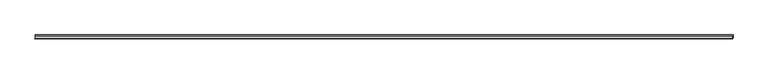
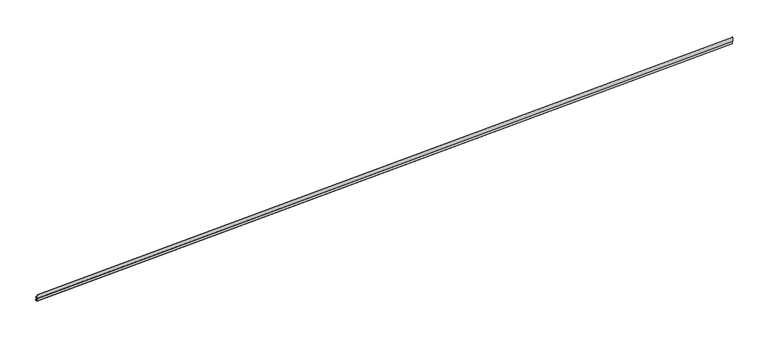
"""IFC4 building model written with IfcOpenShell, lengths in millimetres: proxy geometry, Generic Models 2:Generic Models 2:310765:Generic Models 2:310765 : Generic Models 2:Generic Models 2:310765:197 : Generic Models 2:Generic Models 2:310765:Generic Models 2:310765 : Generic Models 2:Generic Models 2:310765:300385."""

from ifc_helpers import new_model, si_unit, frame, origin, place, context, project, spatial, polyline, outline, extrude, source, transform, mapped, element, save


def generic_models_54930a4b(model_context):
    return source(origin(), model_context, "Body", "SweptSolid", [
        extrude(outline(polyline([(-6.35, 0.0), (-6.35, -90.4875), (-7.9375, -90.4875), (-7.9375, -1.5874999), (-72.095064, -1.5874999), (-72.095064, 11.1125), (-53.045064, 11.1125), (-53.045064, 9.525), (-70.507564, 9.525), (-70.507564, 0.0), (-6.35, 0.0)])), frame((563227.6289933, -578787.9663841, 4134.5272352), z_axis=(0.9991330730923568, 0.0, 0.04163054471206784), x_axis=(0.0, -1.0, 0.0)), (0.0, 0.0, 1.0), 15852.9020761),
        extrude(outline(polyline([(-48.7009311, 5.5562501), (-48.7009311, 56.35625), (-47.1134311, 56.35625), (-47.1134311, 3.96875), (-67.5700628, 3.96875), (-67.5700628, 5.5562501), (-48.7009311, 5.5562501)])), frame((563227.6289933, -578787.9663841, 4134.5272352), z_axis=(0.9991330730923568, 0.0, 0.04163054471206784), x_axis=(0.0, -1.0, 0.0)), (0.0, 0.0, 1.0), 15852.9020761),
        extrude(outline(polyline([(-36.5125, 89.69375), (-36.5125, 26.1937501), (-38.1, 26.1937501), (-38.1, 88.10625), (-97.7325628, 88.10625), (-97.7325628, 89.69375), (-36.5125, 89.69375)])), frame((563227.6289933, -578787.9663841, 4134.5272352), z_axis=(0.9991330730923568, 0.0, 0.04163054471206784), x_axis=(0.0, -1.0, 0.0)), (0.0, 0.0, 1.0), 15852.9020761),
    ])


if __name__ == "__main__":
    model = new_model("IFC4")
    model_context = context("Model", 3, world=origin())
    ifc_project = project(units=[si_unit("LENGTHUNIT", "METRE", prefix="MILLI")], contexts=[model_context])
    site = spatial("IfcSite", under=ifc_project)
    building = spatial("IfcBuilding", under=site)
    placement = place(None, origin())
    generic_models_shape = generic_models_54930a4b(model_context)
    element("IfcBuildingElementProxy", 1, Name="Generic Models 2:Generic Models 2:310765:Generic Models 2:310765 : Generic Models 2:Generic Models 2:310765:197 : Generic Models 2:Generic Models 2:310765:Generic Models 2:310765 : Generic Models 2:Generic Models 2:310765:300385", ObjectType="Generic Models 2:Generic Models 2:310765:Generic Models 2:310765 : Generic Models 2:Generic Models 2:310765:197 : Generic Models 2:Generic Models 2:310765:Generic Models 2:310765 : Generic Models 2:Generic Models 2:310765:300385", at=placement, inside=building, context=model_context, shape_type="MappedRepresentation", body=[
        mapped(generic_models_shape, transform((0.0, 0.0, 0.0), x_axis=(1.0, 0.0, 0.0), y_axis=(0.0, 1.0, 0.0), z_axis=(0.0, 0.0, 1.0))),
    ])
    save(model, "model.ifc")

# Revit data of these elements
# Type "Generic Models 2:Generic Models 2:310765:Generic Models 2:310765 : Generic Models 2:Generic Models 2:310765:197 : Generic Models 2:Generic Models 2:310765:Generic Models 2:310765 : Generic Models 2:Generic Models 2:310765:300385"
#   NameOverride = "Generic Models 2:Generic Models 2:310765:Generic Models 2:310765 : Generic Models 2:Generic Models 2:310765:300385"
#   ObjectTypeOverride = "Generic Models 2:310765 : Generic Models 2:Generic Models 2:310765"
#   Reference = "Generic Models 2"
#   Tag = "300385"
# Element 1 (IfcBuildingElementProxy, "Generic Models 2:Generic Models 2:310765:Generic Models 2:310765 : Generic Models 2:Generic Models 2:310765:197 : Generic Models 2:Generic Models 2:310765:Generic Models 2:310765 : Generic Models 2:Generic Models 2:310765:300385")
#   Materials on its faces: "BRAKE METAL COUNTERFLASHING"
# Materials
#   "BRAKE METAL COUNTERFLASHING": class "Unassigned", colour RGB 210 209 208, transparency 0, Cost = 0
